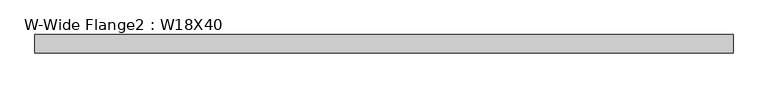
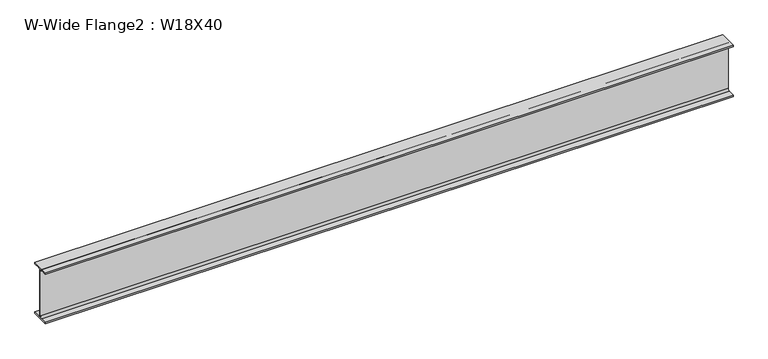
"""IFC4 building model written with IfcOpenShell, lengths in millimetres: beam geometry, W-Wide Flange2 : W18X40."""

import ifcopenshell
import ifcopenshell.guid

model = None  # the IFC model being written
_history = None  # IfcOwnerHistory: only IFC2X3 demands one
_inside = {}  # id of a spatial element -> (the spatial element, [elements in it])
_under = {}  # id of a project, library or spatial element -> (it, [spatial elements below it])
_declared = {}  # id of a project -> (the project, [libraries it declares])
_typed = {}  # id of a type object -> (the type object, [elements of that type])
_made_of = {}  # id of a material, layer set ... -> (it, [elements and type objects made of it])


def new_model(schema):
    """Start an empty IFC model of exactly this schema.

    Asked for "IFC4X3", IfcOpenShell would pick the latest addendum, in which some entities
    have other attributes; the version numbers below select the first issue.
    IFC2X3 requires an IfcOwnerHistory on every rooted entity: one is made here for all.
    """
    global model, _history
    if schema == "IFC4X3":
        model = ifcopenshell.file(schema_version=(4, 3, 0, 0))
    else:
        model = ifcopenshell.file(schema=schema)
    _inside.clear()
    _under.clear()
    _declared.clear()
    _typed.clear()
    _made_of.clear()
    _history = None
    if model.schema == "IFC2X3":
        org = make("IfcOrganization", Name="unknown")
        user = make(
            "IfcPersonAndOrganization",
            ThePerson=make("IfcPerson", FamilyName="unknown"),
            TheOrganization=org,
        )
        app = make(
            "IfcApplication",
            ApplicationDeveloper=org,
            Version="unknown",
            ApplicationFullName="unknown",
            ApplicationIdentifier="unknown",
        )
        _history = make(
            "IfcOwnerHistory",
            OwningUser=user,
            OwningApplication=app,
            ChangeAction="ADDED",
            CreationDate=0,
        )
    return model


def make(cls, **values):
    """One entity of the class cls with the attributes given. An attribute that is None is left unset."""
    return model.create_entity(
        cls, **{name: value for name, value in values.items() if value is not None}
    )


def rooted(cls, **values):
    """An entity with a GlobalId (a new one), such as an element, a storey or a relation."""
    return make(cls, GlobalId=ifcopenshell.guid.new(), OwnerHistory=_history, **values)


def si_unit(unit_type, name, prefix=None):
    """IfcSIUnit, for example si_unit("LENGTHUNIT", "METRE", prefix="MILLI")."""
    return make("IfcSIUnit", UnitType=unit_type, Prefix=prefix, Name=name)


def assignment(units):
    """IfcUnitAssignment: the units of a project."""
    return None if units is None else make("IfcUnitAssignment", Units=units)


def point(xyz):
    """IfcCartesianPoint."""
    return None if xyz is None else make("IfcCartesianPoint", Coordinates=xyz)


def direction(xyz):
    """IfcDirection."""
    return None if xyz is None else make("IfcDirection", DirectionRatios=xyz)


def frame(location, z_axis=None, x_axis=None):
    """IfcAxis2Placement3D, a coordinate frame: its origin and axes. An axis left out is left unset."""
    return make(
        "IfcAxis2Placement3D",
        Location=point(location),
        Axis=direction(z_axis),
        RefDirection=direction(x_axis),
    )


def frame_2d(location, x_axis=None):
    """IfcAxis2Placement2D, a coordinate frame in the plane: its origin and x axis."""
    return make(
        "IfcAxis2Placement2D", Location=point(location), RefDirection=direction(x_axis)
    )


def origin():
    """The frame at (0, 0, 0) with its axes left unset."""
    return frame((0.0, 0.0, 0.0))


def place(relative_to, where):
    """IfcLocalPlacement: puts the frame where relative to a parent placement (None: the world)."""
    return make(
        "IfcLocalPlacement", PlacementRelTo=relative_to, RelativePlacement=where
    )


def context(
    kind, dimensions, precision=None, world=None, true_north=None, identifier=None
):
    """IfcGeometricRepresentationContext, for example the 3D "Model" context."""
    return make(
        "IfcGeometricRepresentationContext",
        ContextIdentifier=identifier,
        ContextType=kind,
        CoordinateSpaceDimension=dimensions,
        Precision=precision,
        WorldCoordinateSystem=world,
        TrueNorth=true_north,
    )


def project(units=None, contexts=None):
    """IfcProject with its units and contexts."""
    return rooted(
        "IfcProject",
        Name="project",
        RepresentationContexts=contexts,
        UnitsInContext=assignment(units),
    )


def spatial(cls, under=None, at=None, **own):
    """A site, building, storey or space (cls), placed at a placement, below another one or the project."""
    s = rooted(cls, ObjectPlacement=at, **own)
    if under is not None:
        _under.setdefault(under.id(), (under, []))[1].append(s)
    return s


def polyline(points):
    """IfcPolyline through the points."""
    return make("IfcPolyline", Points=[point(p) for p in points])


def circle_curve(where, radius):
    """IfcCircle in the frame where."""
    return make("IfcCircle", Position=where, Radius=radius)


def trimmed(basis, trim1, trim2, sense, master):
    """IfcTrimmedCurve: the piece of a basis curve between two trims."""
    return make(
        "IfcTrimmedCurve",
        BasisCurve=basis,
        Trim1=trim1,
        Trim2=trim2,
        SenseAgreement=sense,
        MasterRepresentation=master,
    )


def segment(curve, same_sense, transition):
    """IfcCompositeCurveSegment."""
    return make(
        "IfcCompositeCurveSegment",
        Transition=transition,
        SameSense=same_sense,
        ParentCurve=curve,
    )


def composite_curve(segments, self_intersect=None):
    """IfcCompositeCurve: segments joined end to end."""
    return make("IfcCompositeCurve", Segments=segments, SelfIntersect=self_intersect)


def outline(outer, holes=None, kind="AREA"):
    """IfcArbitraryClosedProfileDef: a profile drawn as a closed curve; with holes, ...WithVoids."""
    if holes is None:
        return make("IfcArbitraryClosedProfileDef", ProfileType=kind, OuterCurve=outer)
    return make(
        "IfcArbitraryProfileDefWithVoids",
        ProfileType=kind,
        OuterCurve=outer,
        InnerCurves=holes,
    )


def extrude(swept, where, along, depth):
    """IfcExtrudedAreaSolid: the profile swept, set in the frame where, extruded along a direction by depth."""
    return make(
        "IfcExtrudedAreaSolid",
        SweptArea=swept,
        Position=where,
        ExtrudedDirection=direction(along),
        Depth=depth,
    )


def shape(context_of_items, identifier, shape_type, items):
    """IfcShapeRepresentation: the items that make up one representation, for example the "Body"."""
    return make(
        "IfcShapeRepresentation",
        ContextOfItems=context_of_items,
        RepresentationIdentifier=identifier,
        RepresentationType=shape_type,
        Items=items,
    )


def source(mapping_origin, context_of_items, identifier, shape_type, items):
    """IfcRepresentationMap: a shape defined once, which mapped items show again and again."""
    return make(
        "IfcRepresentationMap",
        MappingOrigin=mapping_origin,
        MappedRepresentation=shape(context_of_items, identifier, shape_type, items),
    )


def transform(
    local_origin,
    x_axis=None,
    y_axis=None,
    z_axis=None,
    scale=None,
    scale2=None,
    scale3=None,
    uniform=True,
):
    """IfcCartesianTransformationOperator3D, or its non-uniform kind. x_axis, y_axis, z_axis: its Axis1, 2, 3."""
    if uniform:
        return make(
            "IfcCartesianTransformationOperator3D",
            Axis1=direction(x_axis),
            Axis2=direction(y_axis),
            LocalOrigin=point(local_origin),
            Scale=scale,
            Axis3=direction(z_axis),
        )
    return make(
        "IfcCartesianTransformationOperator3DnonUniform",
        Axis1=direction(x_axis),
        Axis2=direction(y_axis),
        LocalOrigin=point(local_origin),
        Scale=scale,
        Axis3=direction(z_axis),
        Scale2=scale2,
        Scale3=scale3,
    )


def mapped(mapping_source, mapping_target):
    """IfcMappedItem: shows the shape of a source again, moved by a transform."""
    return make(
        "IfcMappedItem", MappingSource=mapping_source, MappingTarget=mapping_target
    )


def made_of(thing, what):
    """Note that an element or type object is made of a material, layer set ...; save() writes the relation."""
    if what is not None:
        _made_of.setdefault(what.id(), (what, []))[1].append(thing)
    return thing


def element(
    cls,
    number,
    at=None,
    inside=None,
    cuts=None,
    type_object=None,
    material=None,
    context=None,
    identifier="Body",
    shape_type=None,
    held_by="IfcProductDefinitionShape",
    body=None,
    shapes=None,
    **own,
):
    """One element of the class cls, such as IfcWall. Its Tag is "e" and its number.

    at: its placement. inside: the storey or other place that contains it. cuts: it is an
    opening in that element (IfcRelVoidsElement). A single representation is given by context,
    identifier, shape_type and body (its items); several are given by shapes. held_by: the class
    of the entity that holds the representations. save() writes the other relations.
    """
    e = rooted(cls, Tag="e%d" % number, ObjectPlacement=at, **own)
    if body is not None:
        shapes = [shape(context, identifier, shape_type, body)]
    if shapes is not None:
        e.Representation = make(held_by, Representations=shapes)
    if inside is not None:
        _inside.setdefault(inside.id(), (inside, []))[1].append(e)
    if cuts is not None:
        rooted(
            "IfcRelVoidsElement", RelatingBuildingElement=cuts, RelatedOpeningElement=e
        )
    if type_object is not None:
        _typed.setdefault(type_object.id(), (type_object, []))[1].append(e)
    return made_of(e, material)


def aggregate(whole, parts):
    """IfcRelAggregates: a whole, such as a stair, and the parts it consists of."""
    return rooted("IfcRelAggregates", RelatingObject=whole, RelatedObjects=parts)


def save(model, path):
    """Write the relations noted so far, then the file.

    IfcRelAggregates (storeys below a building ...), IfcRelContainedInSpatialStructure (elements
    in a storey), IfcRelDefinesByType, IfcRelAssociatesMaterial and IfcRelDeclares: one each for
    every whole, place, type object, material and project.
    """
    for whole, parts in _under.values():
        aggregate(whole, parts)
    for where, things in _inside.values():
        rooted(
            "IfcRelContainedInSpatialStructure",
            RelatedElements=things,
            RelatingStructure=where,
        )
    for kind, things in _typed.values():
        rooted("IfcRelDefinesByType", RelatedObjects=things, RelatingType=kind)
    for what, things in _made_of.values():
        rooted("IfcRelAssociatesMaterial", RelatedObjects=things, RelatingMaterial=what)
    for by, libraries in _declared.values():
        rooted("IfcRelDeclares", RelatingContext=by, RelatedDefinitions=libraries)
    model.write(path)


def w_wide_flange2_w18x40_ca46fc5e(model_context):
    return source(origin(), model_context, "Body", "SweptSolid", [
        extrude(outline(composite_curve([segment(polyline([(76.454, -213.995), (76.454, -227.33), (-76.454, -227.33), (-76.454, -213.995), (-20.828, -213.995)]), True, "CONTINUOUS"), segment(trimmed(circle_curve(frame_2d((-20.828, -197.1675)), 16.8275), [point((-20.828, -213.995))], [point((-4.0005, -197.1675))], True, "CARTESIAN"), True, "CONTINUOUS"), segment(polyline([(-4.0005, -197.1675), (-4.0005, 197.1675)]), True, "CONTINUOUS"), segment(trimmed(circle_curve(frame_2d((-20.828, 197.1675)), 16.8275), [point((-4.0005, 197.1675))], [point((-20.828, 213.995))], True, "CARTESIAN"), True, "CONTINUOUS"), segment(polyline([(-20.828, 213.995), (-76.454, 213.995), (-76.454, 227.33), (76.454, 227.33), (76.454, 213.995), (20.828, 213.995)]), True, "CONTINUOUS"), segment(trimmed(circle_curve(frame_2d((20.828, 197.1675)), 16.8275), [point((20.828, 213.995))], [point((4.0005, 197.1675))], True, "CARTESIAN"), True, "CONTINUOUS"), segment(polyline([(4.0005, 197.1675), (4.0005, -197.1675)]), True, "CONTINUOUS"), segment(trimmed(circle_curve(frame_2d((20.828, -197.1675)), 16.8275), [point((4.0005, -197.1675))], [point((20.828, -213.995))], True, "CARTESIAN"), True, "CONTINUOUS"), segment(polyline([(20.828, -213.995), (76.454, -213.995)]), True, "CONTINUOUS")], self_intersect=False)), frame((-2876.153125, 0.0, 0.0), z_axis=(1.0, 0.0, 0.0), x_axis=(0.0, 1.0, 0.0)), (0.0, 0.0, 1.0), 5757.465625),
    ])


if __name__ == "__main__":
    model = new_model("IFC4")
    model_context = context("Model", 3, world=origin())
    ifc_project = project(units=[si_unit("LENGTHUNIT", "METRE", prefix="MILLI")], contexts=[model_context])
    site = spatial("IfcSite", under=ifc_project)
    building = spatial("IfcBuilding", under=site)
    placement = place(None, origin())
    w_wide_flange2_w18x40_shape = w_wide_flange2_w18x40_ca46fc5e(model_context)
    element("IfcBeam", 1, ObjectType="W-Wide Flange2 : W18X40", at=placement, inside=building, context=model_context, shape_type="MappedRepresentation", body=[
        mapped(w_wide_flange2_w18x40_shape, transform((0.0, 0.0, 0.0), x_axis=(1.0, 0.0, 0.0), y_axis=(0.0, 1.0, 0.0), z_axis=(0.0, 0.0, 1.0))),
    ])
    save(model, "model.ifc")

# Revit data of these elements
# Type "W-Wide Flange2 : W18X40"
#   Assembly Code = "B10"
#   W = 40
#   Length [instance default] = 5' - 0"
#   bf = 0' - 6.02"
#   d = 1' - 5.9"
#   k = 0' - 1 3/16"
#   k2 = 0' - 0.6625"
#   tf = 0' - 0.525"
#   tw = 0' - 0.315"
#   A = 0.0819444 SF
#   Structural Material [instance default] = Steel ASTM A992
# Element 1 (IfcBeam, "W-Wide Flange2 : W18X40")
#   Materials on its faces: "Steel ASTM A992"
# Materials
#   "Steel ASTM A992": class "Metal", colour RGB 199 199 199, transparency 0, Description = "Structural steel 50ksi", Cost = 0
